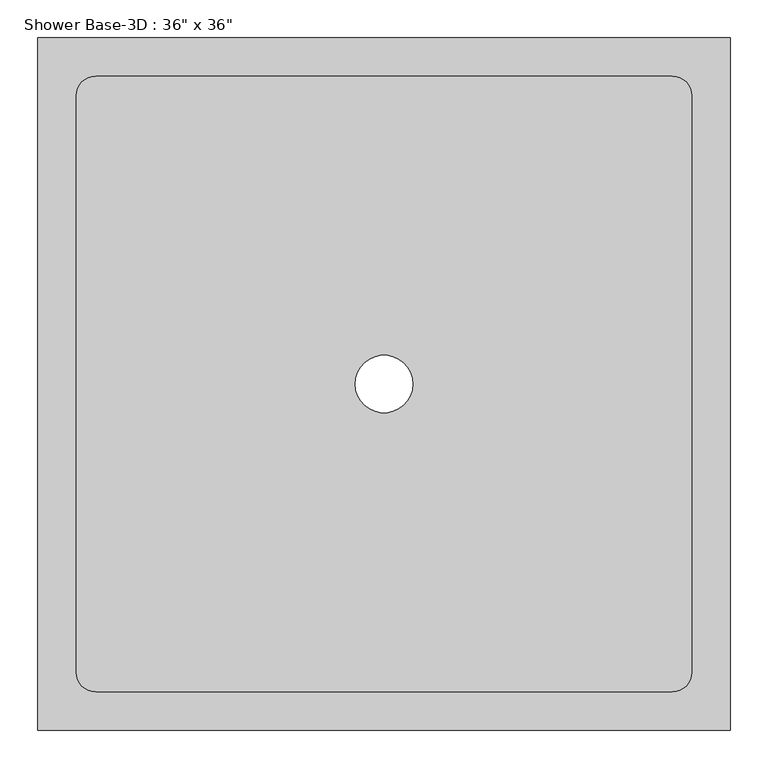
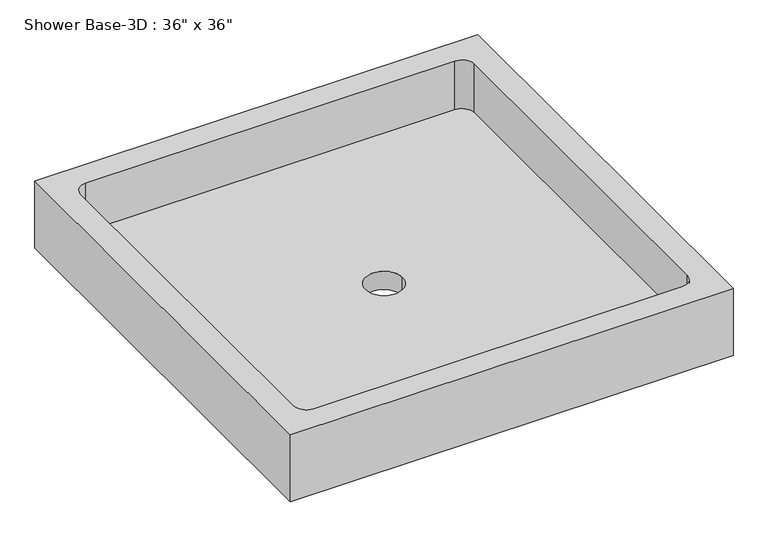
"""IFC4 building model written with IfcOpenShell, lengths in millimetres: flow terminal geometry."""

from ifc_helpers import new_model, si_unit, frame, origin, origin_with_axes, place, context, project, spatial, polyline, circle_curve, source, transform, mapped, element, save
from ifc_brep_helpers import plane_surface, revolved_surface, advanced_brep


def flow_terminal_54cced83(model_context):
    return source(origin(), model_context, "Body", "AdvancedBrep", [
        advanced_brep(
        [(457.2, 457.2, 146.05), (-457.2, 457.2, 146.05), (-457.2, -457.2, 146.05), (457.2, -457.2, 146.05), (406.4, -381.0, 146.05), (381.0, -406.4, 146.05), (-381.0, -406.4, 146.05), (-406.4, -381.0, 146.05), (-406.4, 381.0, 146.05), (-381.0, 406.4, 146.05), (381.0, 406.4, 146.05), (406.4, 381.0, 146.05), (457.2, 457.2, 0.0), (457.2, -457.2, 0.0), (-457.2, -457.2, 0.0), (-457.2, 457.2, 0.0), (-38.1, 0.0, 0.0), (38.1, 0.0, 0.0), (381.0, -406.4, 39.8652193), (406.4, -381.0, 39.8652193), (406.4, 381.0, 39.8652193), (381.0, 406.4, 39.8652193), (-381.0, 406.4, 39.8652193), (-406.4, 381.0, 39.8652193), (-406.4, -381.0, 39.8652193), (-381.0, -406.4, 39.8652193), (38.1, 0.0, 39.8652193), (-38.1, 0.0, 39.8652193)],
        [
            (0, 1),
            (1, 2),
            (2, 3),
            (3, 0),
            (4, 5, circle_curve(frame((381.0, -381.0, 146.05), z_axis=(0.0, 0.0, -1.0), x_axis=(1.0, 0.0, 0.0)), 25.4)),
            (5, 6),
            (6, 7, circle_curve(frame((-381.0, -381.0, 146.05), z_axis=(0.0, 0.0, -1.0), x_axis=(1.0, 0.0, 0.0)), 25.4)),
            (7, 8),
            (8, 9, circle_curve(frame((-381.0, 381.0, 146.05), z_axis=(0.0, 0.0, -1.0), x_axis=(1.0, 0.0, 0.0)), 25.4)),
            (9, 10),
            (10, 11, circle_curve(frame((381.0, 381.0, 146.05), z_axis=(0.0, 0.0, -1.0), x_axis=(1.0, 0.0, 0.0)), 25.4)),
            (11, 4),
            (12, 13),
            (13, 14),
            (14, 15),
            (15, 12),
            (16, 17, circle_curve(origin_with_axes(), 38.1)),
            (17, 16, circle_curve(origin_with_axes(), 38.1)),
            (0, 12),
            (15, 1),
            (14, 2),
            (13, 3),
            (18, 19, circle_curve(frame((381.0, -381.0, 39.8652193), z_axis=(0.0, 0.0, 1.0), x_axis=(1.0, 0.0, 0.0)), 25.4)),
            (19, 20),
            (20, 21, circle_curve(frame((381.0, 381.0, 39.8652193), z_axis=(0.0, 0.0, 1.0), x_axis=(1.0, 0.0, 0.0)), 25.4)),
            (21, 22),
            (22, 23, circle_curve(frame((-381.0, 381.0, 39.8652193), z_axis=(0.0, 0.0, 1.0), x_axis=(1.0, 0.0, 0.0)), 25.4)),
            (23, 24),
            (24, 25, circle_curve(frame((-381.0, -381.0, 39.8652193), z_axis=(0.0, 0.0, 1.0), x_axis=(1.0, 0.0, 0.0)), 25.4)),
            (25, 18),
            (26, 27, circle_curve(frame((0.0, 0.0, 39.8652193), z_axis=(0.0, 0.0, -1.0), x_axis=(1.0, 0.0, 0.0)), 38.1)),
            (27, 26, circle_curve(frame((0.0, 0.0, 39.8652193), z_axis=(0.0, 0.0, -1.0), x_axis=(1.0, 0.0, 0.0)), 38.1)),
            (18, 5),
            (4, 19),
            (11, 20),
            (10, 21),
            (9, 22),
            (8, 23),
            (7, 24),
            (6, 25),
            (16, 27),
            (26, 17),
        ],
        [
            plane_surface(frame((-457.2, 457.2, 146.05), z_axis=(0.0, 0.0, 1.0), x_axis=(-1.0, 0.0, 0.0))),
            plane_surface(frame((-457.2, 457.2, 0.0), z_axis=(0.0, 0.0, -1.0), x_axis=(1.0, 0.0, 0.0))),
            plane_surface(frame((457.2, 457.2, 146.05), z_axis=(0.0, 1.0, 0.0), x_axis=(0.0, 0.0, -1.0))),
            plane_surface(frame((-457.2, 457.2, 146.05), z_axis=(-1.0, 0.0, 0.0), x_axis=(0.0, 0.0, -1.0))),
            plane_surface(frame((-457.2, -457.2, 146.05), z_axis=(0.0, -1.0, 0.0), x_axis=(0.0, 0.0, -1.0))),
            plane_surface(frame((457.2, -457.2, 146.05), z_axis=(1.0, 0.0, 0.0), x_axis=(0.0, 0.0, -1.0))),
            plane_surface(frame((406.4, -381.0, 39.8652193), z_axis=(0.0, 0.0, 1.0), x_axis=(0.0, -1.0, 0.0))),
            revolved_surface(polyline([(406.4, -381.0, 146.05), (406.4, -381.0, 39.8652193)]), (381.0, -381.0, 39.8652193), (0.0, 0.0, 1.0)),
            plane_surface(frame((406.4, -381.0, 146.05), z_axis=(-1.0, 0.0, 0.0), x_axis=(0.0, 0.0, -1.0))),
            revolved_surface(polyline([(406.4, 381.0, 146.05), (406.4, 381.0, 39.8652193)]), (381.0, 381.0, 39.8652193), (0.0, 0.0, 1.0)),
            plane_surface(frame((381.0, 406.4, 146.05), z_axis=(0.0, -1.0, 0.0), x_axis=(0.0, 0.0, -1.0))),
            revolved_surface(polyline([(-355.6, 381.0, 146.05), (-355.6, 381.0, 39.8652193)]), (-381.0, 381.0, 39.8652193), (0.0, 0.0, 1.0)),
            plane_surface(frame((-406.4, 381.0, 146.05), z_axis=(1.0, 0.0, 0.0), x_axis=(0.0, 0.0, -1.0))),
            revolved_surface(polyline([(-355.6, -381.0, 146.05), (-355.6, -381.0, 39.8652193)]), (-381.0, -381.0, 39.8652193), (0.0, 0.0, 1.0)),
            plane_surface(frame((-381.0, -406.4, 146.05), z_axis=(0.0, 1.0, 0.0), x_axis=(0.0, 0.0, -1.0))),
            revolved_surface(polyline([(38.1, 0.0, 39.8652193), (38.1, 0.0, 0.0)]), (0.0, 0.0, 0.0), (0.0, 0.0, 1.0)),
        ],
        [
            (0, [[1, 2, 3, 4], [5, 6, 7, 8, 9, 10, 11, 12]]),
            (1, [[13, 14, 15, 16], [17, 18]]),
            (2, [[-1, 19, -16, 20]]),
            (3, [[-2, -20, -15, 21]]),
            (4, [[-3, -21, -14, 22]]),
            (5, [[-4, -22, -13, -19]]),
            (6, [[23, 24, 25, 26, 27, 28, 29, 30], [31, 32]]),
            (7, [[-23, 33, -5, 34]]),
            (8, [[-24, -34, -12, 35]]),
            (9, [[-25, -35, -11, 36]]),
            (10, [[-26, -36, -10, 37]]),
            (11, [[-27, -37, -9, 38]]),
            (12, [[-28, -38, -8, 39]]),
            (13, [[-29, -39, -7, 40]]),
            (14, [[-30, -40, -6, -33]]),
            (15, [[41, -31, 42, -17]]),
            (15, [[-41, -18, -42, -32]]),
        ],
    ),
    ])


if __name__ == "__main__":
    model = new_model("IFC4")
    model_context = context("Model", 3, world=origin())
    ifc_project = project(units=[si_unit("LENGTHUNIT", "METRE", prefix="MILLI")], contexts=[model_context])
    site = spatial("IfcSite", under=ifc_project)
    building = spatial("IfcBuilding", under=site)
    placement = place(None, origin())
    flow_terminal_shape = flow_terminal_54cced83(model_context)
    element("IfcFlowTerminal", 1, ObjectType="Shower Base-3D : 36\" x 36\"", at=placement, inside=building, context=model_context, shape_type="MappedRepresentation", body=[
        mapped(flow_terminal_shape, transform((0.0, 0.0, 0.0), x_axis=(1.0, 0.0, 0.0), y_axis=(0.0, 1.0, 0.0), z_axis=(0.0, 0.0, 1.0))),
    ])
    save(model, "model.ifc")

# Revit data of these elements
# Type "Shower Base-3D : 36\" x 36\""
#   Assembly Code = "D2010710"
#   Depth = 3' - 0"
#   Width = 3' - 0"
#   Shower Base Material = Laminate, Linen, Matte
#   Default Elevation = 0
# Element 1 (IfcFlowTerminal, "Shower Base-3D : 36\" x 36\"")
#   Materials on its faces: "Laminate, Linen, Matte"
# Materials
#   "Laminate, Linen, Matte": class "Plastic", colour RGB 198 189 176, transparency 0, Description = "Plastic Laminate - Linen, Matte", Cost = 0
